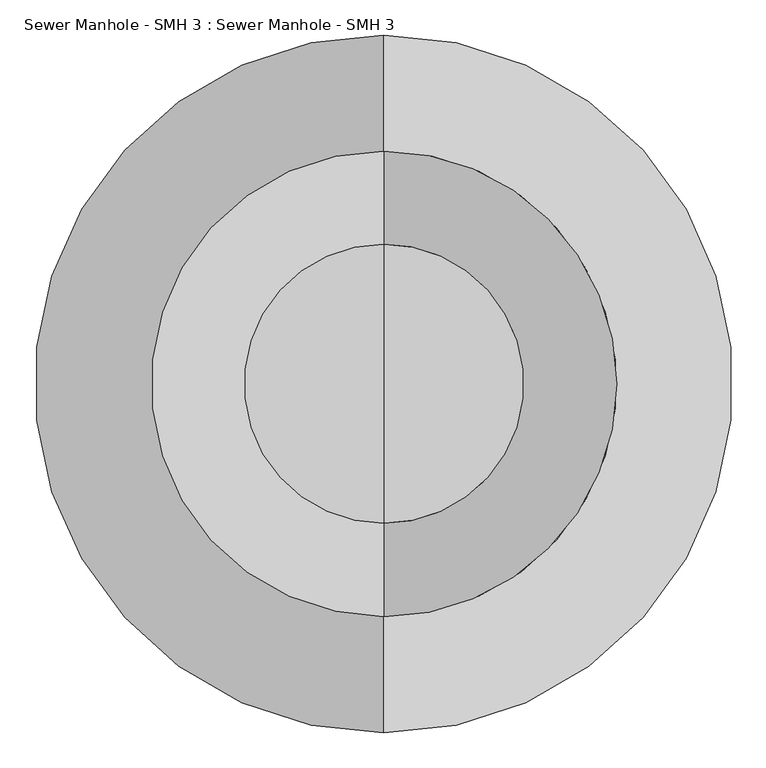
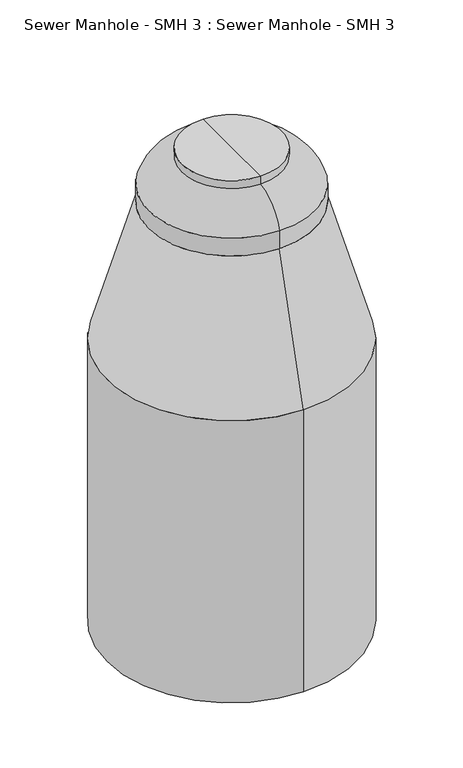
"""IFC4 building model written with IfcOpenShell, lengths in millimetres: proxy geometry, Sewer Manhole - SMH 3 : Sewer Manhole - SMH 3."""

from ifc_helpers import new_model, si_unit, point, frame, origin, place, context, project, spatial, polyline, circle_curve, ellipse_curve, trimmed, source, transform, mapped, element, save
from ifc_brep_helpers import plane_surface, cylinder_surface, revolved_surface, advanced_brep


def sewer_manhole_smh_3_sewer_manhole_smh_3_9c91e7ca(model_context):
    return source(origin(), model_context, "Body", "AdvancedBrep", [
        advanced_brep(
        [(0.0, -508.0, 2704.3270774), (0.0, 508.0, 2704.3270774), (0.0, -762.0, 1818.64), (0.0, 762.0, 1818.64)],
        [
            (0, 1, circle_curve(frame((0.0, 0.0, 2704.3270774), z_axis=(0.0, 0.0, 1.0), x_axis=(0.0, -1.0, 0.0)), 508.0)),
            (1, 0, circle_curve(frame((0.0, 0.0, 2704.3270774), z_axis=(0.0, 0.0, 1.0), x_axis=(0.0, 1.0, 0.0)), 508.0)),
            (2, 3, circle_curve(frame((0.0, 0.0, 1818.64), z_axis=(0.0, 0.0, -1.0), x_axis=(0.0, 1.0, 0.0)), 762.0)),
            (3, 2, circle_curve(frame((0.0, 0.0, 1818.64), z_axis=(0.0, 0.0, -1.0), x_axis=(0.0, -1.0, 0.0)), 762.0)),
            (3, 1),
            (0, 2),
        ],
        [
            plane_surface(frame((0.0, 0.0, 2704.3270774), z_axis=(0.0, 0.0, 1.0), x_axis=(1.0, 0.0, 0.0))),
            plane_surface(frame((0.0, 0.0, 1818.64), z_axis=(0.0, 0.0, -1.0), x_axis=(1.0, 0.0, 0.0))),
            revolved_surface(polyline([(0.0, -508.0000000095596, 2704.3270774), (0.0, -762.0, 1818.6400000000003)]), (0.0, 0.0, 4475.7012323), (0.0, 0.0, -1.0)),
            revolved_surface(polyline([(0.0, 508.0000000095596, 2704.3270774), (0.0, 762.0, 1818.6400000000003)]), (0.0, 0.0, 4475.7012323), (0.0, 0.0, -1.0)),
        ],
        [
            (0, [[1, 2]]),
            (1, [[3, 4]]),
            (2, [[-4, 5, -1, 6]]),
            (3, [[-3, -6, -2, -5]]),
        ],
    ),
        advanced_brep(
        [(0.0, -508.0, 2704.3270774), (0.0, 508.0, 2704.3270774), (0.0, 0.0, 2704.3270774), (0.0, -508.0, 2819.4), (0.0, 508.0, 2819.4), (0.0, -304.8, 2997.2), (0.0, 304.8, 2997.2), (0.0, -304.8, 3048.0), (0.0, 304.8, 3048.0), (0.0, 0.0, 3048.0)],
        [
            (0, 1, circle_curve(frame((0.0, 0.0, 2704.3270774), z_axis=(0.0, 0.0, -1.0), x_axis=(0.0, 1.0, 0.0)), 508.0)),
            (1, 2),
            (2, 0),
            (1, 0, circle_curve(frame((0.0, 0.0, 2704.3270774), z_axis=(0.0, 0.0, -1.0), x_axis=(0.0, 1.0, 0.0)), 508.0)),
            (3, 4, circle_curve(frame((0.0, 0.0, 2819.4), z_axis=(0.0, 0.0, -1.0), x_axis=(0.0, 1.0, 0.0)), 508.0)),
            (4, 1),
            (0, 3),
            (4, 3, circle_curve(frame((0.0, 0.0, 2819.4), z_axis=(0.0, 0.0, -1.0), x_axis=(0.0, 1.0, 0.0)), 508.0)),
            (5, 6, circle_curve(frame((0.0, 0.0, 2997.2), z_axis=(0.0, 0.0, -1.0), x_axis=(0.0, 1.0, 0.0)), 304.8)),
            (6, 4, circle_curve(frame((0.0, 259.6539436, 2740.5902213), z_axis=(-1.0, 0.0, 0.0), x_axis=(0.0, -1.0, 0.0)), 260.550849)),
            (3, 5, circle_curve(frame((0.0, -259.6539436, 2740.5902213), z_axis=(-1.0, 0.0, 0.0), x_axis=(0.0, 1.0, 0.0)), 260.550849)),
            (6, 5, circle_curve(frame((0.0, 0.0, 2997.2), z_axis=(0.0, 0.0, -1.0), x_axis=(0.0, 1.0, 0.0)), 304.8)),
            (7, 8, circle_curve(frame((0.0, 0.0, 3048.0), z_axis=(0.0, 0.0, -1.0), x_axis=(0.0, 1.0, 0.0)), 304.8)),
            (8, 6),
            (5, 7),
            (8, 7, circle_curve(frame((0.0, 0.0, 3048.0), z_axis=(0.0, 0.0, -1.0), x_axis=(0.0, 1.0, 0.0)), 304.8)),
            (9, 8),
            (7, 9),
        ],
        [
            plane_surface(frame((0.0, 0.0, 2704.3270774), z_axis=(0.0, 0.0, -1.0), x_axis=(0.0, 1.0, 0.0))),
            cylinder_surface(frame((0.0, 0.0, 2768.6), z_axis=(0.0, 0.0, 1.0), x_axis=(0.0, 1.0, 0.0)), 508.0),
            revolved_surface(trimmed(ellipse_curve(frame((0.0, 259.6539436, 2740.5902213), z_axis=(1.0, 0.0, 0.0), x_axis=(0.0, -1.0, 0.0)), 260.550849, 260.550849), [point((0.0, 508.0, 2819.4))], [point((0.0, 304.8, 2997.2))], True, "CARTESIAN"), (0.0, 0.0, 2768.6), (0.0, 0.0, 1.0)),
            cylinder_surface(frame((0.0, 0.0, 2768.6), z_axis=(0.0, 0.0, 1.0), x_axis=(0.0, 1.0, 0.0)), 304.8),
            plane_surface(frame((0.0, 0.0, 3048.0), z_axis=(0.0, 0.0, 1.0), x_axis=(0.0, 1.0, 0.0))),
        ],
        [
            (0, [[1, 2, 3]]),
            (0, [[4, -3, -2]]),
            (1, [[5, 6, -1, 7]]),
            (1, [[8, -7, -4, -6]]),
            (2, [[9, 10, -5, 11]]),
            (2, [[12, -11, -8, -10]]),
            (3, [[13, 14, -9, 15]]),
            (3, [[16, -15, -12, -14]]),
            (4, [[17, -13, 18]]),
            (4, [[-18, -16, -17]]),
        ],
    ),
        advanced_brep(
        [(0.0, -762.0, 1818.64), (0.0, 762.0, 1818.64), (0.0, 762.0, 0.0), (0.0, -762.0, 0.0), (0.0, 0.0, 0.0), (0.0, 0.0, 1818.64)],
        [
            (0, 1, circle_curve(frame((0.0, 0.0, 1818.64), z_axis=(0.0, 0.0, -1.0), x_axis=(0.0, 1.0, 0.0)), 762.0)),
            (1, 2),
            (2, 3, circle_curve(frame((0.0, 0.0, 0.0), z_axis=(0.0, 0.0, 1.0), x_axis=(0.0, 1.0, 0.0)), 762.0)),
            (3, 0),
            (1, 0, circle_curve(frame((0.0, 0.0, 1818.64), z_axis=(0.0, 0.0, -1.0), x_axis=(0.0, 1.0, 0.0)), 762.0)),
            (3, 2, circle_curve(frame((0.0, 0.0, 0.0), z_axis=(0.0, 0.0, 1.0), x_axis=(0.0, 1.0, 0.0)), 762.0)),
            (2, 4),
            (4, 3),
            (5, 1),
            (0, 5),
        ],
        [
            cylinder_surface(frame((0.0, 0.0, 457.2), z_axis=(0.0, 0.0, 1.0), x_axis=(0.0, 1.0, 0.0)), 762.0),
            plane_surface(frame((0.0, 0.0, 0.0), z_axis=(0.0, 0.0, -1.0), x_axis=(0.0, 1.0, 0.0))),
            plane_surface(frame((0.0, 0.0, 1818.64), z_axis=(0.0, 0.0, 1.0), x_axis=(0.0, 1.0, 0.0))),
        ],
        [
            (0, [[1, 2, 3, 4]]),
            (0, [[5, -4, 6, -2]]),
            (1, [[-3, 7, 8]]),
            (1, [[-6, -8, -7]]),
            (2, [[9, -1, 10]]),
            (2, [[-10, -5, -9]]),
        ],
    ),
    ])


if __name__ == "__main__":
    model = new_model("IFC4")
    model_context = context("Model", 3, world=origin())
    ifc_project = project(units=[si_unit("LENGTHUNIT", "METRE", prefix="MILLI")], contexts=[model_context])
    site = spatial("IfcSite", under=ifc_project)
    building = spatial("IfcBuilding", under=site)
    placement = place(None, origin())
    sewer_manhole_smh_3_sewer_manhole_smh_3_shape = sewer_manhole_smh_3_sewer_manhole_smh_3_9c91e7ca(model_context)
    element("IfcBuildingElementProxy", 1, Name="Sewer Manhole - SMH 3 : Sewer Manhole - SMH 3", ObjectType="Sewer Manhole - SMH 3 : Sewer Manhole - SMH 3", at=placement, inside=building, context=model_context, shape_type="MappedRepresentation", body=[
        mapped(sewer_manhole_smh_3_sewer_manhole_smh_3_shape, transform((0.0, 0.0, 0.0), x_axis=(1.0, 0.0, 0.0), y_axis=(0.0, 1.0, 0.0), z_axis=(0.0, 0.0, 1.0))),
    ])
    save(model, "model.ifc")
